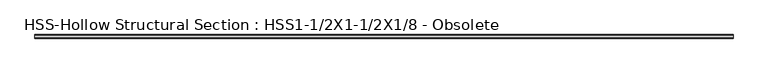
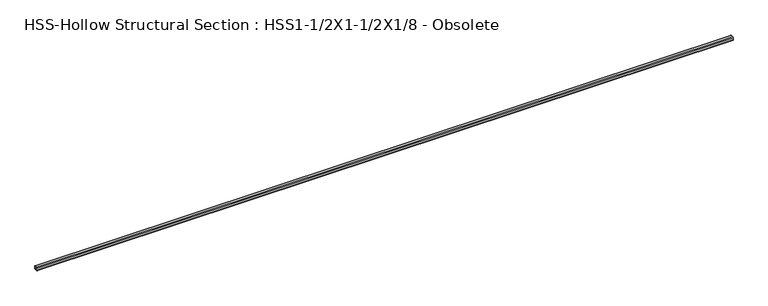
"""IFC4 building model written with IfcOpenShell, lengths in millimetres: beam geometry, HSS-Hollow Structural Section : HSS1-1/2X1-1/2X1/8 - Obsolete."""

import ifcopenshell
import ifcopenshell.guid

model = None  # the IFC model being written
_history = None  # IfcOwnerHistory: only IFC2X3 demands one
_inside = {}  # id of a spatial element -> (the spatial element, [elements in it])
_under = {}  # id of a project, library or spatial element -> (it, [spatial elements below it])
_declared = {}  # id of a project -> (the project, [libraries it declares])
_typed = {}  # id of a type object -> (the type object, [elements of that type])
_made_of = {}  # id of a material, layer set ... -> (it, [elements and type objects made of it])


def new_model(schema):
    """Start an empty IFC model of exactly this schema.

    Asked for "IFC4X3", IfcOpenShell would pick the latest addendum, in which some entities
    have other attributes; the version numbers below select the first issue.
    IFC2X3 requires an IfcOwnerHistory on every rooted entity: one is made here for all.
    """
    global model, _history
    if schema == "IFC4X3":
        model = ifcopenshell.file(schema_version=(4, 3, 0, 0))
    else:
        model = ifcopenshell.file(schema=schema)
    _inside.clear()
    _under.clear()
    _declared.clear()
    _typed.clear()
    _made_of.clear()
    _history = None
    if model.schema == "IFC2X3":
        org = make("IfcOrganization", Name="unknown")
        user = make(
            "IfcPersonAndOrganization",
            ThePerson=make("IfcPerson", FamilyName="unknown"),
            TheOrganization=org,
        )
        app = make(
            "IfcApplication",
            ApplicationDeveloper=org,
            Version="unknown",
            ApplicationFullName="unknown",
            ApplicationIdentifier="unknown",
        )
        _history = make(
            "IfcOwnerHistory",
            OwningUser=user,
            OwningApplication=app,
            ChangeAction="ADDED",
            CreationDate=0,
        )
    return model


def make(cls, **values):
    """One entity of the class cls with the attributes given. An attribute that is None is left unset."""
    return model.create_entity(
        cls, **{name: value for name, value in values.items() if value is not None}
    )


def rooted(cls, **values):
    """An entity with a GlobalId (a new one), such as an element, a storey or a relation."""
    return make(cls, GlobalId=ifcopenshell.guid.new(), OwnerHistory=_history, **values)


def si_unit(unit_type, name, prefix=None):
    """IfcSIUnit, for example si_unit("LENGTHUNIT", "METRE", prefix="MILLI")."""
    return make("IfcSIUnit", UnitType=unit_type, Prefix=prefix, Name=name)


def assignment(units):
    """IfcUnitAssignment: the units of a project."""
    return None if units is None else make("IfcUnitAssignment", Units=units)


def point(xyz):
    """IfcCartesianPoint."""
    return None if xyz is None else make("IfcCartesianPoint", Coordinates=xyz)


def direction(xyz):
    """IfcDirection."""
    return None if xyz is None else make("IfcDirection", DirectionRatios=xyz)


def frame(location, z_axis=None, x_axis=None):
    """IfcAxis2Placement3D, a coordinate frame: its origin and axes. An axis left out is left unset."""
    return make(
        "IfcAxis2Placement3D",
        Location=point(location),
        Axis=direction(z_axis),
        RefDirection=direction(x_axis),
    )


def frame_2d(location, x_axis=None):
    """IfcAxis2Placement2D, a coordinate frame in the plane: its origin and x axis."""
    return make(
        "IfcAxis2Placement2D", Location=point(location), RefDirection=direction(x_axis)
    )


def origin():
    """The frame at (0, 0, 0) with its axes left unset."""
    return frame((0.0, 0.0, 0.0))


def place(relative_to, where):
    """IfcLocalPlacement: puts the frame where relative to a parent placement (None: the world)."""
    return make(
        "IfcLocalPlacement", PlacementRelTo=relative_to, RelativePlacement=where
    )


def context(
    kind, dimensions, precision=None, world=None, true_north=None, identifier=None
):
    """IfcGeometricRepresentationContext, for example the 3D "Model" context."""
    return make(
        "IfcGeometricRepresentationContext",
        ContextIdentifier=identifier,
        ContextType=kind,
        CoordinateSpaceDimension=dimensions,
        Precision=precision,
        WorldCoordinateSystem=world,
        TrueNorth=true_north,
    )


def project(units=None, contexts=None):
    """IfcProject with its units and contexts."""
    return rooted(
        "IfcProject",
        Name="project",
        RepresentationContexts=contexts,
        UnitsInContext=assignment(units),
    )


def spatial(cls, under=None, at=None, **own):
    """A site, building, storey or space (cls), placed at a placement, below another one or the project."""
    s = rooted(cls, ObjectPlacement=at, **own)
    if under is not None:
        _under.setdefault(under.id(), (under, []))[1].append(s)
    return s


def polyline(points):
    """IfcPolyline through the points."""
    return make("IfcPolyline", Points=[point(p) for p in points])


def circle_curve(where, radius):
    """IfcCircle in the frame where."""
    return make("IfcCircle", Position=where, Radius=radius)


def trimmed(basis, trim1, trim2, sense, master):
    """IfcTrimmedCurve: the piece of a basis curve between two trims."""
    return make(
        "IfcTrimmedCurve",
        BasisCurve=basis,
        Trim1=trim1,
        Trim2=trim2,
        SenseAgreement=sense,
        MasterRepresentation=master,
    )


def segment(curve, same_sense, transition):
    """IfcCompositeCurveSegment."""
    return make(
        "IfcCompositeCurveSegment",
        Transition=transition,
        SameSense=same_sense,
        ParentCurve=curve,
    )


def composite_curve(segments, self_intersect=None):
    """IfcCompositeCurve: segments joined end to end."""
    return make("IfcCompositeCurve", Segments=segments, SelfIntersect=self_intersect)


def outline(outer, holes=None, kind="AREA"):
    """IfcArbitraryClosedProfileDef: a profile drawn as a closed curve; with holes, ...WithVoids."""
    if holes is None:
        return make("IfcArbitraryClosedProfileDef", ProfileType=kind, OuterCurve=outer)
    return make(
        "IfcArbitraryProfileDefWithVoids",
        ProfileType=kind,
        OuterCurve=outer,
        InnerCurves=holes,
    )


def extrude(swept, where, along, depth):
    """IfcExtrudedAreaSolid: the profile swept, set in the frame where, extruded along a direction by depth."""
    return make(
        "IfcExtrudedAreaSolid",
        SweptArea=swept,
        Position=where,
        ExtrudedDirection=direction(along),
        Depth=depth,
    )


def shape(context_of_items, identifier, shape_type, items):
    """IfcShapeRepresentation: the items that make up one representation, for example the "Body"."""
    return make(
        "IfcShapeRepresentation",
        ContextOfItems=context_of_items,
        RepresentationIdentifier=identifier,
        RepresentationType=shape_type,
        Items=items,
    )


def source(mapping_origin, context_of_items, identifier, shape_type, items):
    """IfcRepresentationMap: a shape defined once, which mapped items show again and again."""
    return make(
        "IfcRepresentationMap",
        MappingOrigin=mapping_origin,
        MappedRepresentation=shape(context_of_items, identifier, shape_type, items),
    )


def transform(
    local_origin,
    x_axis=None,
    y_axis=None,
    z_axis=None,
    scale=None,
    scale2=None,
    scale3=None,
    uniform=True,
):
    """IfcCartesianTransformationOperator3D, or its non-uniform kind. x_axis, y_axis, z_axis: its Axis1, 2, 3."""
    if uniform:
        return make(
            "IfcCartesianTransformationOperator3D",
            Axis1=direction(x_axis),
            Axis2=direction(y_axis),
            LocalOrigin=point(local_origin),
            Scale=scale,
            Axis3=direction(z_axis),
        )
    return make(
        "IfcCartesianTransformationOperator3DnonUniform",
        Axis1=direction(x_axis),
        Axis2=direction(y_axis),
        LocalOrigin=point(local_origin),
        Scale=scale,
        Axis3=direction(z_axis),
        Scale2=scale2,
        Scale3=scale3,
    )


def mapped(mapping_source, mapping_target):
    """IfcMappedItem: shows the shape of a source again, moved by a transform."""
    return make(
        "IfcMappedItem", MappingSource=mapping_source, MappingTarget=mapping_target
    )


def made_of(thing, what):
    """Note that an element or type object is made of a material, layer set ...; save() writes the relation."""
    if what is not None:
        _made_of.setdefault(what.id(), (what, []))[1].append(thing)
    return thing


def element(
    cls,
    number,
    at=None,
    inside=None,
    cuts=None,
    type_object=None,
    material=None,
    context=None,
    identifier="Body",
    shape_type=None,
    held_by="IfcProductDefinitionShape",
    body=None,
    shapes=None,
    **own,
):
    """One element of the class cls, such as IfcWall. Its Tag is "e" and its number.

    at: its placement. inside: the storey or other place that contains it. cuts: it is an
    opening in that element (IfcRelVoidsElement). A single representation is given by context,
    identifier, shape_type and body (its items); several are given by shapes. held_by: the class
    of the entity that holds the representations. save() writes the other relations.
    """
    e = rooted(cls, Tag="e%d" % number, ObjectPlacement=at, **own)
    if body is not None:
        shapes = [shape(context, identifier, shape_type, body)]
    if shapes is not None:
        e.Representation = make(held_by, Representations=shapes)
    if inside is not None:
        _inside.setdefault(inside.id(), (inside, []))[1].append(e)
    if cuts is not None:
        rooted(
            "IfcRelVoidsElement", RelatingBuildingElement=cuts, RelatedOpeningElement=e
        )
    if type_object is not None:
        _typed.setdefault(type_object.id(), (type_object, []))[1].append(e)
    return made_of(e, material)


def aggregate(whole, parts):
    """IfcRelAggregates: a whole, such as a stair, and the parts it consists of."""
    return rooted("IfcRelAggregates", RelatingObject=whole, RelatedObjects=parts)


def save(model, path):
    """Write the relations noted so far, then the file.

    IfcRelAggregates (storeys below a building ...), IfcRelContainedInSpatialStructure (elements
    in a storey), IfcRelDefinesByType, IfcRelAssociatesMaterial and IfcRelDeclares: one each for
    every whole, place, type object, material and project.
    """
    for whole, parts in _under.values():
        aggregate(whole, parts)
    for where, things in _inside.values():
        rooted(
            "IfcRelContainedInSpatialStructure",
            RelatedElements=things,
            RelatingStructure=where,
        )
    for kind, things in _typed.values():
        rooted("IfcRelDefinesByType", RelatedObjects=things, RelatingType=kind)
    for what, things in _made_of.values():
        rooted("IfcRelAssociatesMaterial", RelatedObjects=things, RelatingMaterial=what)
    for by, libraries in _declared.values():
        rooted("IfcRelDeclares", RelatingContext=by, RelatedDefinitions=libraries)
    model.write(path)


def hss_hollow_structural_section_hss1_1_2x1_1_2x1_8_obsolete_55b26b90(model_context):
    return source(origin(), model_context, "Body", "SweptSolid", [
        extrude(outline(composite_curve([segment(polyline([(19.05, 13.1572), (19.05, -13.1572)]), True, "CONTINUOUS"), segment(trimmed(circle_curve(frame_2d((13.1572, -13.1572)), 5.8928), [point((19.05, -13.1572))], [point((13.1572, -19.05))], False, "CARTESIAN"), True, "CONTINUOUS"), segment(polyline([(13.1572, -19.05), (-13.1572, -19.05)]), True, "CONTINUOUS"), segment(trimmed(circle_curve(frame_2d((-13.1572, -13.1572)), 5.8928), [point((-13.1572, -19.05))], [point((-19.05, -13.1572))], False, "CARTESIAN"), True, "CONTINUOUS"), segment(polyline([(-19.05, -13.1572), (-19.05, 13.1572)]), True, "CONTINUOUS"), segment(trimmed(circle_curve(frame_2d((-13.1572, 13.1572)), 5.8928), [point((-19.05, 13.1572))], [point((-13.1572, 19.05))], False, "CARTESIAN"), True, "CONTINUOUS"), segment(polyline([(-13.1572, 19.05), (13.1572, 19.05)]), True, "CONTINUOUS"), segment(trimmed(circle_curve(frame_2d((13.1572, 13.1572)), 5.8928), [point((13.1572, 19.05))], [point((19.05, 13.1572))], False, "CARTESIAN"), True, "CONTINUOUS")], self_intersect=False), holes=[composite_curve([segment(trimmed(circle_curve(frame_2d((-13.1572, 13.1572)), 2.9464), [point((-13.1572, 16.1036))], [point((-16.1036, 13.1572))], True, "CARTESIAN"), True, "CONTINUOUS"), segment(polyline([(-16.1036, 13.1572), (-16.1036, -13.1572)]), True, "CONTINUOUS"), segment(trimmed(circle_curve(frame_2d((-13.1572, -13.1572)), 2.9464), [point((-16.1036, -13.1572))], [point((-13.1572, -16.1036))], True, "CARTESIAN"), True, "CONTINUOUS"), segment(polyline([(-13.1572, -16.1036), (13.1572, -16.1036)]), True, "CONTINUOUS"), segment(trimmed(circle_curve(frame_2d((13.1572, -13.1572)), 2.9464), [point((13.1572, -16.1036))], [point((16.1036, -13.1572))], True, "CARTESIAN"), True, "CONTINUOUS"), segment(polyline([(16.1036, -13.1572), (16.1036, 13.1572)]), True, "CONTINUOUS"), segment(trimmed(circle_curve(frame_2d((13.1572, 13.1572)), 2.9464), [point((16.1036, 13.1572))], [point((13.1572, 16.1036))], True, "CARTESIAN"), True, "CONTINUOUS"), segment(polyline([(13.1572, 16.1036), (-13.1572, 16.1036)]), True, "CONTINUOUS")], self_intersect=False)]), frame((-3675.0625, 0.0, 0.0), z_axis=(1.0, 0.0, 0.0), x_axis=(0.0, 1.0, 0.0)), (0.0, 0.0, 1.0), 7350.125),
    ])


if __name__ == "__main__":
    model = new_model("IFC4")
    model_context = context("Model", 3, world=origin())
    ifc_project = project(units=[si_unit("LENGTHUNIT", "METRE", prefix="MILLI")], contexts=[model_context])
    site = spatial("IfcSite", under=ifc_project)
    building = spatial("IfcBuilding", under=site)
    placement = place(None, origin())
    hss_hollow_structural_section_hss1_1_2x1_1_2x1_8_obsolete_shape = hss_hollow_structural_section_hss1_1_2x1_1_2x1_8_obsolete_55b26b90(model_context)
    element("IfcBeam", 1, ObjectType="HSS-Hollow Structural Section : HSS1-1/2X1-1/2X1/8 - Obsolete", at=placement, inside=building, context=model_context, shape_type="MappedRepresentation", body=[
        mapped(hss_hollow_structural_section_hss1_1_2x1_1_2x1_8_obsolete_shape, transform((0.0, 0.0, 0.0), x_axis=(1.0, 0.0, 0.0), y_axis=(0.0, 1.0, 0.0), z_axis=(0.0, 0.0, 1.0))),
    ])
    save(model, "model.ifc")

# Revit data of these elements
# Type "HSS-Hollow Structural Section : HSS1-1/2X1-1/2X1/8 - Obsolete"
#   Assembly Code = "B10"
#   Shape = "Square"
#   W = 2.19
#   Ht = 0' - 1 1/2"
#   Length [instance default] = 5' - 0"
#   b = 0' - 1 1/2"
#   kr = 0' - 0.232"
#   t = 0' - 0.116"
#   A = 0.00423611 SF
#   Structural Material [instance default] = 1 1/2" X 1 1/2" x 1/8" ALUM. TUBE
# Element 1 (IfcBeam, "HSS-Hollow Structural Section : HSS1-1/2X1-1/2X1/8 - Obsolete")
#   Materials on its faces: "1 1/2\" X 1 1/2\" x 1/8\" ALUM. TUBE"
# Materials
#   "1 1/2\" X 1 1/2\" x 1/8\" ALUM. TUBE": class "Metal", colour RGB 199 199 199, transparency 0, Description = "Carbon steel", Cost = 0
